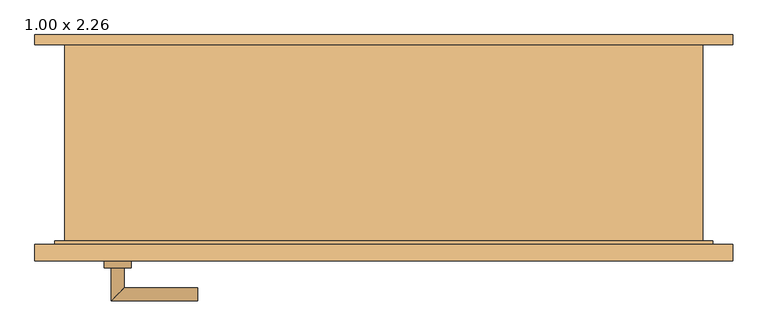
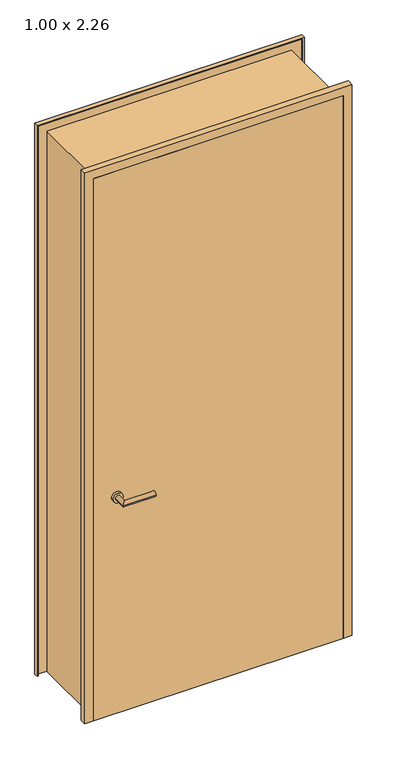
"""IFC4 building model written with IfcOpenShell, lengths in millimetres: door geometry, Drehflügel 1-flg - Stahlzarge : 1.00 x 2.26."""

from ifc_helpers import new_model, si_unit, point, frame, frame_2d, origin, place, context, project, spatial, polyline, circle_curve, ellipse_curve, trimmed, segment, composite_curve, outline, extrude, faceted_brep, source, transform, mapped, element, save
from ifc_brep_helpers import plane_surface, cylinder_surface, advanced_brep


def door_1_00_x_2_26_9a2ce12e(model_context):
    return source(origin(), model_context, "Body", "SolidModel", [
        advanced_brep(
        [(-410.0, -139.4346141, 1000.0), (-390.0, -139.4346141, 1000.0), (-390.0, -89.4346141, 1000.0), (-410.0, -69.4346141, 1000.0), (-280.0, -69.4346141, 1000.0), (-280.0, -89.4346141, 1000.0)],
        [
            (0, 1, circle_curve(frame((-400.0, -139.4346141, 1000.0), z_axis=(0.0, -1.0, 0.0), x_axis=(1.0, 0.0, 0.0)), 10.0)),
            (1, 0, circle_curve(frame((-400.0, -139.4346141, 1000.0), z_axis=(0.0, -1.0, 0.0), x_axis=(1.0, 0.0, 0.0)), 10.0)),
            (1, 2),
            (2, 3, ellipse_curve(frame((-400.0, -79.4346141, 1000.0), z_axis=(-0.7071067811865385, -0.7071067811865565, 0.0), x_axis=(0.7071067811865563, -0.7071067811865386, 0.0)), 14.1421356, 10.0)),
            (3, 0),
            (3, 2, ellipse_curve(frame((-400.0, -79.4346141, 1000.0), z_axis=(-0.7071067811865385, -0.7071067811865565, 0.0), x_axis=(0.7071067811865563, -0.7071067811865386, 0.0)), 14.1421356, 10.0)),
            (4, 5, circle_curve(frame((-280.0, -79.4346141, 1000.0), z_axis=(1.0, 0.0, 0.0), x_axis=(0.0, -1.0, 0.0)), 10.0)),
            (5, 4, circle_curve(frame((-280.0, -79.4346141, 1000.0), z_axis=(1.0, 0.0, 0.0), x_axis=(0.0, -1.0, 0.0)), 10.0)),
            (2, 5),
            (4, 3),
        ],
        [
            plane_surface(frame((-400.0, -139.4346141, -287.7526403), z_axis=(0.0, -1.0, 0.0), x_axis=(0.0, 0.0, 1.0))),
            cylinder_surface(frame((-400.0, -139.4346141, 1000.0), z_axis=(0.0, -1.0, 0.0), x_axis=(1.0, 0.0, 0.0)), 10.0),
            plane_surface(frame((-280.0, -79.4346141, -287.7526403), z_axis=(1.0, 0.0, 0.0), x_axis=(0.0, 0.0, 1.0))),
            cylinder_surface(frame((-400.0, -79.4346141, 1000.0), z_axis=(-1.0, 0.0, 0.0), x_axis=(0.0, -1.0, 0.0)), 10.0),
        ],
        [
            (0, [[1, 2]]),
            (1, [[3, 4, 5, -2]]),
            (1, [[-5, 6, -3, -1]]),
            (2, [[7, 8]]),
            (3, [[9, -7, 10, -4]]),
            (3, [[-10, -8, -9, -6]]),
        ],
    ),
        advanced_brep(
        [(-390.0, -199.4346141, 1000.0), (-410.0, -199.4346141, 1000.0), (-410.0, -249.4346141, 1000.0), (-390.0, -229.4346141, 1000.0), (-280.0, -229.4346141, 1000.0), (-280.0, -249.4346141, 1000.0)],
        [
            (0, 1, circle_curve(frame((-400.0, -199.4346141, 1000.0), z_axis=(0.0, 1.0, 0.0), x_axis=(-1.0, 0.0, 0.0)), 10.0)),
            (1, 0, circle_curve(frame((-400.0, -199.4346141, 1000.0), z_axis=(0.0, 1.0, 0.0), x_axis=(-1.0, 0.0, 0.0)), 10.0)),
            (1, 2),
            (2, 3, ellipse_curve(frame((-400.0, -239.4346141, 1000.0), z_axis=(-0.7071067811865475, 0.7071067811865475, 0.0), x_axis=(0.7071067811865474, 0.7071067811865476, 0.0)), 14.1421356, 10.0)),
            (3, 0),
            (3, 2, ellipse_curve(frame((-400.0, -239.4346141, 1000.0), z_axis=(-0.7071067811865475, 0.7071067811865475, 0.0), x_axis=(0.7071067811865474, 0.7071067811865476, 0.0)), 14.1421356, 10.0)),
            (4, 5, circle_curve(frame((-280.0, -239.4346141, 1000.0), z_axis=(1.0, 0.0, 0.0), x_axis=(0.0, -1.0, 0.0)), 10.0)),
            (5, 4, circle_curve(frame((-280.0, -239.4346141, 1000.0), z_axis=(1.0, 0.0, 0.0), x_axis=(0.0, -1.0, 0.0)), 10.0)),
            (2, 5),
            (4, 3),
        ],
        [
            plane_surface(frame((-400.0, -199.4346141, -287.7526403), z_axis=(0.0, 1.0, 0.0), x_axis=(0.0, 0.0, 1.0))),
            cylinder_surface(frame((-400.0, -199.4346141, 1000.0), z_axis=(0.0, 1.0, 0.0), x_axis=(-1.0, 0.0, 0.0)), 10.0),
            plane_surface(frame((-280.0, -239.4346141, -287.7526403), z_axis=(1.0, 0.0, 0.0), x_axis=(0.0, 0.0, 1.0))),
            cylinder_surface(frame((-400.0, -239.4346141, 1000.0), z_axis=(-1.0, 0.0, 0.0), x_axis=(0.0, -1.0, 0.0)), 10.0),
        ],
        [
            (0, [[1, 2]]),
            (1, [[3, 4, 5, -2]]),
            (1, [[-5, 6, -3, -1]]),
            (2, [[7, 8]]),
            (3, [[9, -7, 10, -4]]),
            (3, [[-10, -8, -9, -6]]),
        ],
    ),
        extrude(outline(composite_curve([segment(trimmed(circle_curve(frame_2d((1000.0, -400.0)), 20.0), [point((1000.0, -420.0))], [point((1000.0, -380.0))], False, "CARTESIAN"), True, "CONTINUOUS"), segment(trimmed(circle_curve(frame_2d((1000.0, -400.0)), 20.0), [point((1000.0, -380.0))], [point((1000.0, -420.0))], False, "CARTESIAN"), True, "CONTINUOUS")], self_intersect=False)), frame((0.0, -139.4346141, 0.0), z_axis=(0.0, 1.0, 0.0), x_axis=(0.0, 0.0, 1.0)), (0.0, 0.0, 1.0), 10.0),
        extrude(outline(composite_curve([segment(trimmed(circle_curve(frame_2d((1000.0, -400.0)), 20.0), [point((1000.0, -420.0))], [point((1000.0, -380.0))], False, "CARTESIAN"), True, "CONTINUOUS"), segment(trimmed(circle_curve(frame_2d((1000.0, -400.0)), 20.0), [point((1000.0, -380.0))], [point((1000.0, -420.0))], False, "CARTESIAN"), True, "CONTINUOUS")], self_intersect=False)), frame((0.0, -199.4346141, 0.0), z_axis=(0.0, 1.0, 0.0), x_axis=(0.0, 0.0, 1.0)), (0.0, 0.0, 1.0), 10.0),
        extrude(outline(polyline([(490.0, -164.4346141), (490.0, -189.4346141), (-490.0, -189.4346141), (-490.0, -164.4346141), (490.0, -164.4346141)])), frame((0.0, 0.0, 100.0), z_axis=(0.0, 0.0, 1.0), x_axis=(1.0, 0.0, 0.0)), (0.0, 0.0, 1.0), 2250.0),
        faceted_brep([(524.4603207, 150.5653859, 100.0), (524.4603207, 135.5653859, 100.0), (519.4603207, 135.5653859, 100.0), (519.4603207, 145.5653859, 100.0), (480.0, 145.5653859, 100.0), (480.0, -159.4346141, 100.0), (495.0, -159.4346141, 100.0), (495.0, -184.4346141, 100.0), (519.4603207, -184.4346141, 100.0), (519.4603207, -164.4346141, 100.0), (524.4603207, -164.4346141, 100.0), (524.4603207, -189.4346141, 100.0), (490.0, -189.4346141, 100.0), (490.0, -164.4346141, 100.0), (475.0, -164.4346141, 100.0), (475.0, 150.5653859, 100.0), (475.0, 150.5653859, 2335.0), (-475.0, 150.5653859, 2335.0), (-475.0, 150.5653859, 100.0), (-524.4603207, 150.5653859, 100.0), (-524.4603207, 150.5653859, 2384.4603207), (524.4603207, 150.5653859, 2384.4603207), (475.0, -164.4346141, 2335.0), (490.0, -164.4346141, 2350.0), (-490.0, -164.4346141, 2350.0), (-490.0, -164.4346141, 100.0), (-475.0, -164.4346141, 100.0), (-475.0, -164.4346141, 2335.0), (490.0, -189.4346141, 2350.0), (524.4603207, -189.4346141, 2384.4603207), (-524.4603207, -189.4346141, 2384.4603207), (-524.4603207, -189.4346141, 100.0), (-490.0, -189.4346141, 100.0), (-490.0, -189.4346141, 2350.0), (524.4603207, -164.4346141, 2384.4603207), (519.4603207, -164.4346141, 2379.4603207), (-519.4603207, -164.4346141, 2379.4603207), (-519.4603207, -164.4346141, 100.0), (-524.4603207, -164.4346141, 100.0), (-524.4603207, -164.4346141, 2384.4603207), (519.4603207, -184.4346141, 2379.4603207), (495.0, -184.4346141, 2355.0), (-495.0, -184.4346141, 2355.0), (-495.0, -184.4346141, 100.0), (-519.4603207, -184.4346141, 100.0), (-519.4603207, -184.4346141, 2379.4603207), (495.0, -159.4346141, 2355.0), (480.0, -159.4346141, 2340.0), (-480.0, -159.4346141, 2340.0), (-480.0, -159.4346141, 100.0), (-495.0, -159.4346141, 100.0), (-495.0, -159.4346141, 2355.0), (480.0, 145.5653859, 2340.0), (519.4603207, 145.5653859, 2379.4603207), (-519.4603207, 145.5653859, 2379.4603207), (-519.4603207, 145.5653859, 100.0), (-480.0, 145.5653859, 100.0), (-480.0, 145.5653859, 2340.0), (519.4603207, 135.5653859, 2379.4603207), (524.4603207, 135.5653859, 2384.4603207), (-524.4603207, 135.5653859, 2384.4603207), (-524.4603207, 135.5653859, 100.0), (-519.4603207, 135.5653859, 100.0), (-519.4603207, 135.5653859, 2379.4603207)], [[[0, 1, 2, 3, 4, 5, 6, 7, 8, 9, 10, 11, 12, 13, 14, 15]], [[15, 16, 17, 18, 19, 20, 21, 0]], [[14, 22, 16, 15]], [[13, 23, 24, 25, 26, 27, 22, 14]], [[12, 28, 23, 13]], [[11, 29, 30, 31, 32, 33, 28, 12]], [[10, 34, 29, 11]], [[9, 35, 36, 37, 38, 39, 34, 10]], [[8, 40, 35, 9]], [[7, 41, 42, 43, 44, 45, 40, 8]], [[6, 46, 41, 7]], [[5, 47, 48, 49, 50, 51, 46, 6]], [[4, 52, 47, 5]], [[3, 53, 54, 55, 56, 57, 52, 4]], [[2, 58, 53, 3]], [[1, 59, 60, 61, 62, 63, 58, 2]], [[0, 21, 59, 1]], [[20, 19, 61, 60]], [[19, 18, 26, 25, 32, 31, 38, 37, 44, 43, 50, 49, 56, 55, 62, 61]], [[27, 26, 18, 17]], [[33, 32, 25, 24]], [[39, 38, 31, 30]], [[45, 44, 37, 36]], [[51, 50, 43, 42]], [[57, 56, 49, 48]], [[63, 62, 55, 54]], [[22, 27, 17, 16]], [[28, 33, 24, 23]], [[34, 39, 30, 29]], [[40, 45, 36, 35]], [[46, 51, 42, 41]], [[52, 57, 48, 47]], [[58, 63, 54, 53]], [[21, 20, 60, 59]]]),
    ])


if __name__ == "__main__":
    model = new_model("IFC4")
    model_context = context("Model", 3, world=origin())
    ifc_project = project(units=[si_unit("LENGTHUNIT", "METRE", prefix="MILLI")], contexts=[model_context])
    site = spatial("IfcSite", under=ifc_project)
    building = spatial("IfcBuilding", under=site)
    placement = place(None, origin())
    door_1_00_x_2_26_shape = door_1_00_x_2_26_9a2ce12e(model_context)
    element("IfcDoor", 1, ObjectType="Drehflügel 1-flg - Stahlzarge : 1.00 x 2.26", at=placement, inside=building, context=model_context, shape_type="MappedRepresentation", body=[
        mapped(door_1_00_x_2_26_shape, transform((0.0, 0.0, 0.0), x_axis=(1.0, 0.0, 0.0), y_axis=(0.0, 1.0, 0.0), z_axis=(0.0, 0.0, 1.0))),
    ])
    save(model, "model.ifc")

# Revit data of these elements
# Type "Drehflügel 1-flg - Stahlzarge : 1.00 x 2.26"
#   Construction Type Id = "MDOOR"
#   Type Mark = "20"
#   Operation = "SingleSwingRight"
#   Keynote = "16.03"
#   Analytic Construction = "Metall"
#   Thermal Resistance (R) = 0.270117 (m²·K)/W
#   Heat Transfer Coefficient (U) = 3.7021 W/(m²·K)
#   Rough Width = 1.000 m
#   Rough Height [instance default] = 2.360 m
#   Höhe Türgriff [instance default] = 0.900 m
#   Height = 2.260 m
#   Fußbodenaufbau [instance default] = 0.100 m
#   Width = 1.000 m
#   Sichtbarkeit Sturzlinien [instance default] = yes
#   Türgriff auswählen [instance default] = element 221079
#   Türgriff [instance default] = none
#   Türflügel [instance default] = none
#   Rahmen/Pfosten [instance default] = Metall - Lackiert - Grau
#   Visual Light Transmittance = 0
#   Solar Heat Gain Coefficient = 0
#   Function = (empty or 0)
#   Wall Closure = (empty or 0)
# Element 1 (IfcDoor, "Drehflügel 1-flg - Stahlzarge : 1.00 x 2.26")
#   Materials on its faces: "Metall - Lackiert - Grau", "Metall - Chrom", "Holz - Birke"
# Materials
#   "Metall - Lackiert - Grau": class "Farbe 1", colour RGB 98 98 98, transparency 0, Cost = 0
#   "Metall - Chrom": class "Metall", colour RGB 247 247 247, transparency 0, Cost = 0
#   "Holz - Birke": class "Holz", colour RGB 213 164 103, transparency 0, Cost = 0
